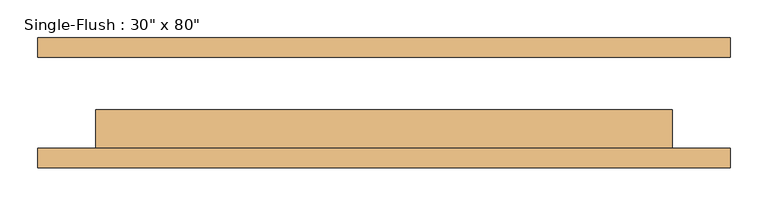
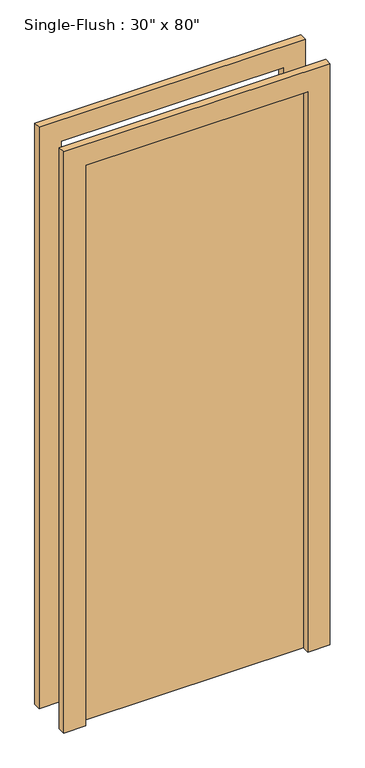
"""IFC4 building model written with IfcOpenShell, lengths in millimetres: door geometry."""

from ifc_helpers import new_model, si_unit, frame, origin, origin_with_axes, place, context, project, spatial, polyline, outline, extrude, source, transform, mapped, element, save


def door_4b3e31f1(model_context):
    return source(origin(), model_context, "Body", "SweptSolid", [
        extrude(outline(polyline([(2108.2, -457.2), (0.0, -457.2), (0.0, -381.0), (2032.0, -381.0), (2032.0, 381.0), (0.0, 381.0), (0.0, 457.2), (2108.2, 457.2), (2108.2, -457.2)])), frame((0.0, -85.725, 0.0), z_axis=(0.0, 1.0, 0.0), x_axis=(0.0, 0.0, 1.0)), (0.0, 0.0, 1.0), 25.4),
        extrude(outline(polyline([(2108.2, 457.2), (2108.2, -457.2), (0.0, -457.2), (0.0, -381.0), (2032.0, -381.0), (2032.0, 381.0), (0.0, 381.0), (0.0, 457.2), (2108.2, 457.2)])), frame((0.0, 60.325, 0.0), z_axis=(0.0, 1.0, 0.0), x_axis=(0.0, 0.0, 1.0)), (0.0, 0.0, 1.0), 25.4),
        extrude(outline(polyline([(381.0, -9.525), (381.0, -60.325), (-381.0, -60.325), (-381.0, -9.525), (381.0, -9.525)])), origin_with_axes(), (0.0, 0.0, 1.0), 2032.0),
    ])


if __name__ == "__main__":
    model = new_model("IFC4")
    model_context = context("Model", 3, world=origin())
    ifc_project = project(units=[si_unit("LENGTHUNIT", "METRE", prefix="MILLI")], contexts=[model_context])
    site = spatial("IfcSite", under=ifc_project)
    building = spatial("IfcBuilding", under=site)
    placement = place(None, origin())
    door_shape = door_4b3e31f1(model_context)
    element("IfcDoor", 1, ObjectType="Single-Flush : 30\" x 80\"", at=placement, inside=building, context=model_context, shape_type="MappedRepresentation", body=[
        mapped(door_shape, transform((0.0, 0.0, 0.0), x_axis=(1.0, 0.0, 0.0), y_axis=(0.0, 1.0, 0.0), z_axis=(0.0, 0.0, 1.0))),
    ])
    save(model, "model.ifc")

# Revit data of these elements
# Type "Single-Flush : 30\" x 80\""
#   Type Mark = "5"
#   Assembly Code = "C1020"
#   Thickness = 0' - 2"
#   Height = 6' - 8"
#   Trim Projection Ext = 0' - 1"
#   Trim Projection Int = 0' - 1"
#   Trim Width = 0' - 3"
#   Width = 2' - 6"
#   Door Material = none
#   Frame Material = none
#   Function = (empty or 0)
#   Wall Closure = (empty or 0)
